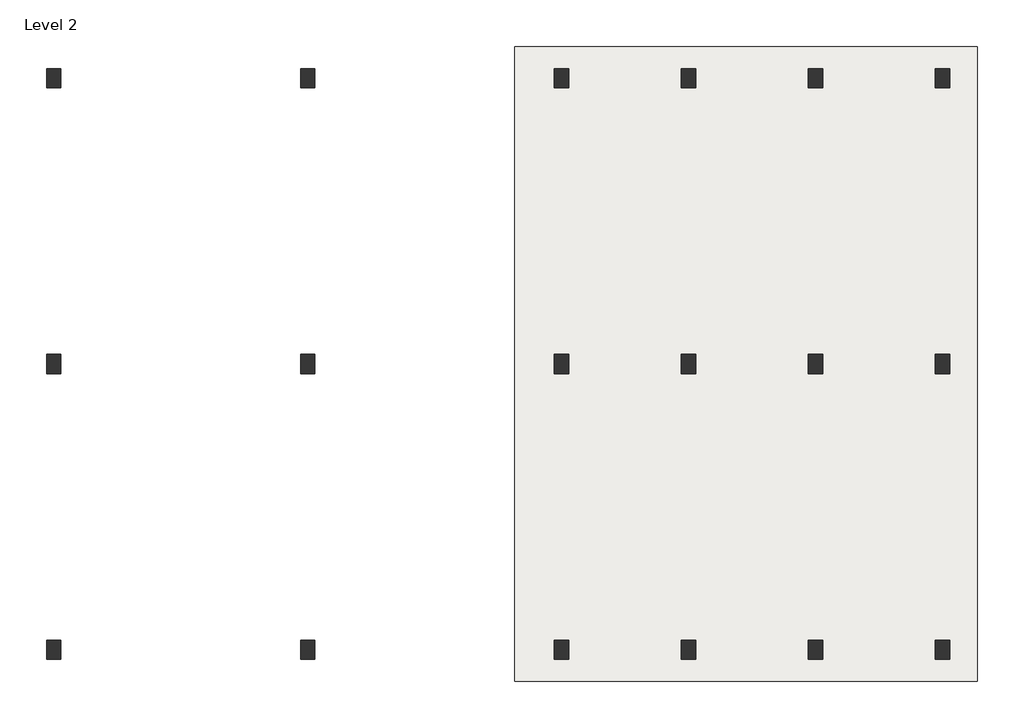
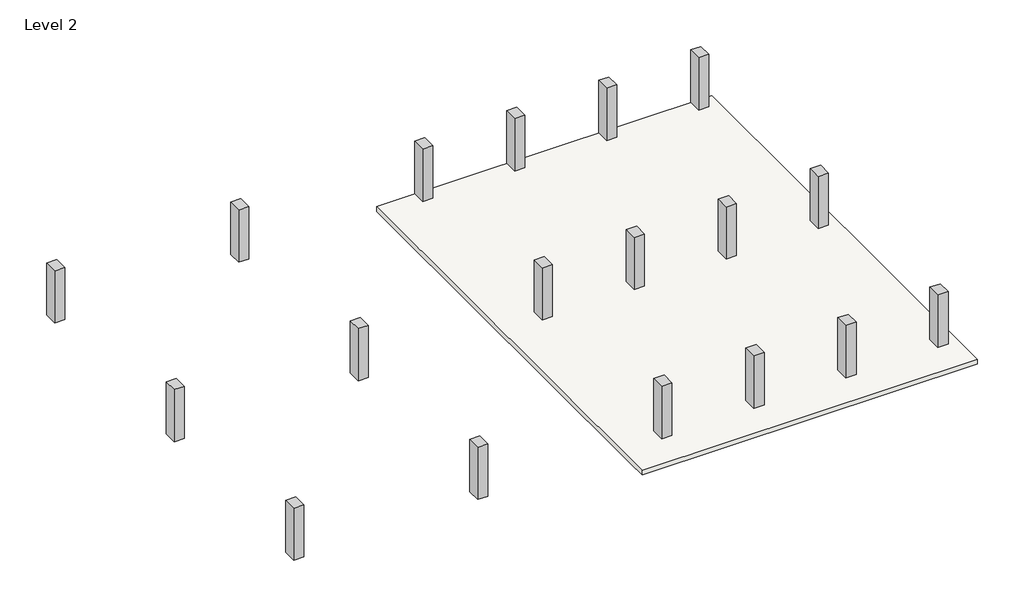
# One storey: 18 columns, 1 slab.
"""IFC4 building model written with IfcOpenShell, lengths in millimetres."""

import ifcopenshell
import ifcopenshell.guid

model = None  # the IFC model being written
_history = None  # IfcOwnerHistory: only IFC2X3 demands one
_inside = {}  # id of a spatial element -> (the spatial element, [elements in it])
_under = {}  # id of a project, library or spatial element -> (it, [spatial elements below it])
_declared = {}  # id of a project -> (the project, [libraries it declares])
_typed = {}  # id of a type object -> (the type object, [elements of that type])
_made_of = {}  # id of a material, layer set ... -> (it, [elements and type objects made of it])


def new_model(schema):
    """Start an empty IFC model of exactly this schema.

    Asked for "IFC4X3", IfcOpenShell would pick the latest addendum, in which some entities
    have other attributes; the version numbers below select the first issue.
    IFC2X3 requires an IfcOwnerHistory on every rooted entity: one is made here for all.
    """
    global model, _history
    if schema == "IFC4X3":
        model = ifcopenshell.file(schema_version=(4, 3, 0, 0))
    else:
        model = ifcopenshell.file(schema=schema)
    _inside.clear()
    _under.clear()
    _declared.clear()
    _typed.clear()
    _made_of.clear()
    _history = None
    if model.schema == "IFC2X3":
        org = make("IfcOrganization", Name="unknown")
        user = make(
            "IfcPersonAndOrganization",
            ThePerson=make("IfcPerson", FamilyName="unknown"),
            TheOrganization=org,
        )
        app = make(
            "IfcApplication",
            ApplicationDeveloper=org,
            Version="unknown",
            ApplicationFullName="unknown",
            ApplicationIdentifier="unknown",
        )
        _history = make(
            "IfcOwnerHistory",
            OwningUser=user,
            OwningApplication=app,
            ChangeAction="ADDED",
            CreationDate=0,
        )
    return model


def make(cls, **values):
    """One entity of the class cls with the attributes given. An attribute that is None is left unset."""
    return model.create_entity(
        cls, **{name: value for name, value in values.items() if value is not None}
    )


def rooted(cls, **values):
    """An entity with a GlobalId (a new one), such as an element, a storey or a relation."""
    return make(cls, GlobalId=ifcopenshell.guid.new(), OwnerHistory=_history, **values)


def si_unit(unit_type, name, prefix=None):
    """IfcSIUnit, for example si_unit("LENGTHUNIT", "METRE", prefix="MILLI")."""
    return make("IfcSIUnit", UnitType=unit_type, Prefix=prefix, Name=name)


def assignment(units):
    """IfcUnitAssignment: the units of a project."""
    return None if units is None else make("IfcUnitAssignment", Units=units)


def point(xyz):
    """IfcCartesianPoint."""
    return None if xyz is None else make("IfcCartesianPoint", Coordinates=xyz)


def direction(xyz):
    """IfcDirection."""
    return None if xyz is None else make("IfcDirection", DirectionRatios=xyz)


def frame(location, z_axis=None, x_axis=None):
    """IfcAxis2Placement3D, a coordinate frame: its origin and axes. An axis left out is left unset."""
    return make(
        "IfcAxis2Placement3D",
        Location=point(location),
        Axis=direction(z_axis),
        RefDirection=direction(x_axis),
    )


def origin():
    """The frame at (0, 0, 0) with its axes left unset."""
    return frame((0.0, 0.0, 0.0))


def place(relative_to, where):
    """IfcLocalPlacement: puts the frame where relative to a parent placement (None: the world)."""
    return make(
        "IfcLocalPlacement", PlacementRelTo=relative_to, RelativePlacement=where
    )


def context(
    kind, dimensions, precision=None, world=None, true_north=None, identifier=None
):
    """IfcGeometricRepresentationContext, for example the 3D "Model" context."""
    return make(
        "IfcGeometricRepresentationContext",
        ContextIdentifier=identifier,
        ContextType=kind,
        CoordinateSpaceDimension=dimensions,
        Precision=precision,
        WorldCoordinateSystem=world,
        TrueNorth=true_north,
    )


def project(units=None, contexts=None):
    """IfcProject with its units and contexts."""
    return rooted(
        "IfcProject",
        Name="project",
        RepresentationContexts=contexts,
        UnitsInContext=assignment(units),
    )


def spatial(cls, under=None, at=None, **own):
    """A site, building, storey or space (cls), placed at a placement, below another one or the project."""
    s = rooted(cls, ObjectPlacement=at, **own)
    if under is not None:
        _under.setdefault(under.id(), (under, []))[1].append(s)
    return s


def polyline(points):
    """IfcPolyline through the points."""
    return make("IfcPolyline", Points=[point(p) for p in points])


def outline(outer, holes=None, kind="AREA"):
    """IfcArbitraryClosedProfileDef: a profile drawn as a closed curve; with holes, ...WithVoids."""
    if holes is None:
        return make("IfcArbitraryClosedProfileDef", ProfileType=kind, OuterCurve=outer)
    return make(
        "IfcArbitraryProfileDefWithVoids",
        ProfileType=kind,
        OuterCurve=outer,
        InnerCurves=holes,
    )


def extrude(swept, where, along, depth):
    """IfcExtrudedAreaSolid: the profile swept, set in the frame where, extruded along a direction by depth."""
    return make(
        "IfcExtrudedAreaSolid",
        SweptArea=swept,
        Position=where,
        ExtrudedDirection=direction(along),
        Depth=depth,
    )


def faces_of(points, faces, orient=None, outer=None):
    """IfcFace entities. A face is a list of loops; a loop is a list of indices into points, from 0.

    orient and outer hold one flag for each loop. By default every Orientation is true, the
    first loop of a face is its IfcFaceOuterBound and the others are IfcFaceBound.
    """
    made = []
    for i, loops in enumerate(faces):
        bounds = []
        for j, loop in enumerate(loops):
            is_outer = j == 0 if outer is None else outer[i][j]
            bounds.append(
                make(
                    "IfcFaceOuterBound" if is_outer else "IfcFaceBound",
                    Bound=make("IfcPolyLoop", Polygon=[points[k] for k in loop]),
                    Orientation=True if orient is None else orient[i][j],
                )
            )
        made.append(make("IfcFace", Bounds=bounds))
    return made


def faceted_brep(points, faces, orient=None, outer=None, voids=None):
    """IfcFacetedBrep: a solid bounded by flat faces; with voids (closed shells), ...WithVoids."""
    shared = [point(p) for p in points]
    hull = make("IfcClosedShell", CfsFaces=faces_of(shared, faces, orient, outer))
    if voids is None:
        return make("IfcFacetedBrep", Outer=hull)
    return make(
        "IfcFacetedBrepWithVoids",
        Outer=hull,
        Voids=[
            make(cls, CfsFaces=faces_of(shared, fs, o, b)) for cls, fs, o, b in voids
        ],
    )


def shape(context_of_items, identifier, shape_type, items):
    """IfcShapeRepresentation: the items that make up one representation, for example the "Body"."""
    return make(
        "IfcShapeRepresentation",
        ContextOfItems=context_of_items,
        RepresentationIdentifier=identifier,
        RepresentationType=shape_type,
        Items=items,
    )


def source(mapping_origin, context_of_items, identifier, shape_type, items):
    """IfcRepresentationMap: a shape defined once, which mapped items show again and again."""
    return make(
        "IfcRepresentationMap",
        MappingOrigin=mapping_origin,
        MappedRepresentation=shape(context_of_items, identifier, shape_type, items),
    )


def transform(
    local_origin,
    x_axis=None,
    y_axis=None,
    z_axis=None,
    scale=None,
    scale2=None,
    scale3=None,
    uniform=True,
):
    """IfcCartesianTransformationOperator3D, or its non-uniform kind. x_axis, y_axis, z_axis: its Axis1, 2, 3."""
    if uniform:
        return make(
            "IfcCartesianTransformationOperator3D",
            Axis1=direction(x_axis),
            Axis2=direction(y_axis),
            LocalOrigin=point(local_origin),
            Scale=scale,
            Axis3=direction(z_axis),
        )
    return make(
        "IfcCartesianTransformationOperator3DnonUniform",
        Axis1=direction(x_axis),
        Axis2=direction(y_axis),
        LocalOrigin=point(local_origin),
        Scale=scale,
        Axis3=direction(z_axis),
        Scale2=scale2,
        Scale3=scale3,
    )


def mapped(mapping_source, mapping_target):
    """IfcMappedItem: shows the shape of a source again, moved by a transform."""
    return make(
        "IfcMappedItem", MappingSource=mapping_source, MappingTarget=mapping_target
    )


def made_of(thing, what):
    """Note that an element or type object is made of a material, layer set ...; save() writes the relation."""
    if what is not None:
        _made_of.setdefault(what.id(), (what, []))[1].append(thing)
    return thing


def element(
    cls,
    number,
    at=None,
    inside=None,
    cuts=None,
    type_object=None,
    material=None,
    context=None,
    identifier="Body",
    shape_type=None,
    held_by="IfcProductDefinitionShape",
    body=None,
    shapes=None,
    **own,
):
    """One element of the class cls, such as IfcWall. Its Tag is "e" and its number.

    at: its placement. inside: the storey or other place that contains it. cuts: it is an
    opening in that element (IfcRelVoidsElement). A single representation is given by context,
    identifier, shape_type and body (its items); several are given by shapes. held_by: the class
    of the entity that holds the representations. save() writes the other relations.
    """
    e = rooted(cls, Tag="e%d" % number, ObjectPlacement=at, **own)
    if body is not None:
        shapes = [shape(context, identifier, shape_type, body)]
    if shapes is not None:
        e.Representation = make(held_by, Representations=shapes)
    if inside is not None:
        _inside.setdefault(inside.id(), (inside, []))[1].append(e)
    if cuts is not None:
        rooted(
            "IfcRelVoidsElement", RelatingBuildingElement=cuts, RelatedOpeningElement=e
        )
    if type_object is not None:
        _typed.setdefault(type_object.id(), (type_object, []))[1].append(e)
    return made_of(e, material)


def aggregate(whole, parts):
    """IfcRelAggregates: a whole, such as a stair, and the parts it consists of."""
    return rooted("IfcRelAggregates", RelatingObject=whole, RelatedObjects=parts)


def save(model, path):
    """Write the relations noted so far, then the file.

    IfcRelAggregates (storeys below a building ...), IfcRelContainedInSpatialStructure (elements
    in a storey), IfcRelDefinesByType, IfcRelAssociatesMaterial and IfcRelDeclares: one each for
    every whole, place, type object, material and project.
    """
    for whole, parts in _under.values():
        aggregate(whole, parts)
    for where, things in _inside.values():
        rooted(
            "IfcRelContainedInSpatialStructure",
            RelatedElements=things,
            RelatingStructure=where,
        )
    for kind, things in _typed.values():
        rooted("IfcRelDefinesByType", RelatedObjects=things, RelatingType=kind)
    for what, things in _made_of.values():
        rooted("IfcRelAssociatesMaterial", RelatedObjects=things, RelatingMaterial=what)
    for by, libraries in _declared.values():
        rooted("IfcRelDeclares", RelatingContext=by, RelatedDefinitions=libraries)
    model.write(path)


def concrete_rectangular_column_450_x_600mm_14788169(model_context):
    return source(origin(), model_context, "Body", "SweptSolid", [
        extrude(outline(polyline([(225.0, 300.0), (225.0, -300.0), (-225.0, -300.0), (-225.0, 300.0), (225.0, 300.0)])), frame((0.0, 0.0, 3600.0), z_axis=(0.0, 0.0, 1.0), x_axis=(1.0, 0.0, 0.0)), (0.0, 0.0, 1.0), 2400.0),
    ])


model = new_model("IFC4")

# Units and contexts
model_context = context("Model", 3, world=origin())
ifc_project = project(units=[si_unit("LENGTHUNIT", "METRE", prefix="MILLI")], contexts=[model_context])

# Site, building, storey
site = spatial("IfcSite", under=ifc_project)
building = spatial("IfcBuilding", under=site)
storey = spatial("IfcBuildingStorey", under=building, Name="Level 2", Elevation=3000.0)

# Columns
placement = place(None, origin())
element("IfcColumn", 1, ObjectType="Concrete-Rectangular-Column : 450 x 600mm", at=placement, inside=storey, context=model_context, shape_type="SweptSolid", body=[
    extrude(outline(polyline([(1008.7948332, 9883.1317199), (1008.7948332, 9283.1317199), (558.7948332, 9283.1317199), (558.7948332, 9883.1317199), (1008.7948332, 9883.1317199)])), frame((0.0, 0.0, 3600.0), z_axis=(0.0, 0.0, 1.0), x_axis=(1.0, 0.0, 0.0)), (0.0, 0.0, 1.0), 2400.0),
])
element("IfcColumn", 2, ObjectType="Concrete-Rectangular-Column : 450 x 600mm", at=placement, inside=storey, context=model_context, shape_type="SweptSolid", body=[
    extrude(outline(polyline([(5008.7948332, 9883.1317199), (5008.7948332, 9283.1317199), (4558.7948332, 9283.1317199), (4558.7948332, 9883.1317199), (5008.7948332, 9883.1317199)])), frame((0.0, 0.0, 3600.0), z_axis=(0.0, 0.0, 1.0), x_axis=(1.0, 0.0, 0.0)), (0.0, 0.0, 1.0), 2400.0),
])
element("IfcColumn", 3, ObjectType="Concrete-Rectangular-Column : 450 x 600mm", at=placement, inside=storey, context=model_context, shape_type="SweptSolid", body=[
    extrude(outline(polyline([(9008.7948332, 9883.1317199), (9008.7948332, 9283.1317199), (8558.7948332, 9283.1317199), (8558.7948332, 9883.1317199), (9008.7948332, 9883.1317199)])), frame((0.0, 0.0, 3600.0), z_axis=(0.0, 0.0, 1.0), x_axis=(1.0, 0.0, 0.0)), (0.0, 0.0, 1.0), 2400.0),
])
element("IfcColumn", 4, ObjectType="Concrete-Rectangular-Column : 450 x 600mm", at=placement, inside=storey, context=model_context, shape_type="SweptSolid", body=[
    extrude(outline(polyline([(13008.7948332, 9883.1317199), (13008.7948332, 9283.1317199), (12558.7948332, 9283.1317199), (12558.7948332, 9883.1317199), (13008.7948332, 9883.1317199)])), frame((0.0, 0.0, 3600.0), z_axis=(0.0, 0.0, 1.0), x_axis=(1.0, 0.0, 0.0)), (0.0, 0.0, 1.0), 2400.0),
])
element("IfcColumn", 5, ObjectType="Concrete-Rectangular-Column : 450 x 600mm", at=placement, inside=storey, context=model_context, shape_type="SweptSolid", body=[
    extrude(outline(polyline([(13008.7948332, 883.1317199), (13008.7948332, 283.1317199), (12558.7948332, 283.1317199), (12558.7948332, 883.1317199), (13008.7948332, 883.1317199)])), frame((0.0, 0.0, 3600.0), z_axis=(0.0, 0.0, 1.0), x_axis=(1.0, 0.0, 0.0)), (0.0, 0.0, 1.0), 2400.0),
])
element("IfcColumn", 6, ObjectType="Concrete-Rectangular-Column : 450 x 600mm", at=placement, inside=storey, context=model_context, shape_type="SweptSolid", body=[
    extrude(outline(polyline([(9008.7948332, 883.1317199), (9008.7948332, 283.1317199), (8558.7948332, 283.1317199), (8558.7948332, 883.1317199), (9008.7948332, 883.1317199)])), frame((0.0, 0.0, 3600.0), z_axis=(0.0, 0.0, 1.0), x_axis=(1.0, 0.0, 0.0)), (0.0, 0.0, 1.0), 2400.0),
])
element("IfcColumn", 7, ObjectType="Concrete-Rectangular-Column : 450 x 600mm", at=placement, inside=storey, context=model_context, shape_type="SweptSolid", body=[
    extrude(outline(polyline([(5008.7948332, 883.1317199), (5008.7948332, 283.1317199), (4558.7948332, 283.1317199), (4558.7948332, 883.1317199), (5008.7948332, 883.1317199)])), frame((0.0, 0.0, 3600.0), z_axis=(0.0, 0.0, 1.0), x_axis=(1.0, 0.0, 0.0)), (0.0, 0.0, 1.0), 2400.0),
])
element("IfcColumn", 8, ObjectType="Concrete-Rectangular-Column : 450 x 600mm", at=placement, inside=storey, context=model_context, shape_type="SweptSolid", body=[
    extrude(outline(polyline([(1008.7948332, 883.1317199), (1008.7948332, 283.1317199), (558.7948332, 283.1317199), (558.7948332, 883.1317199), (1008.7948332, 883.1317199)])), frame((0.0, 0.0, 3600.0), z_axis=(0.0, 0.0, 1.0), x_axis=(1.0, 0.0, 0.0)), (0.0, 0.0, 1.0), 2400.0),
])
element("IfcColumn", 9, ObjectType="Concrete-Rectangular-Column : 450 x 600mm", at=placement, inside=storey, context=model_context, shape_type="SweptSolid", body=[
    extrude(outline(polyline([(1008.7948332, -8116.8682801), (1008.7948332, -8716.8682801), (558.7948332, -8716.8682801), (558.7948332, -8116.8682801), (1008.7948332, -8116.8682801)])), frame((0.0, 0.0, 3600.0), z_axis=(0.0, 0.0, 1.0), x_axis=(1.0, 0.0, 0.0)), (0.0, 0.0, 1.0), 2400.0),
])
element("IfcColumn", 10, ObjectType="Concrete-Rectangular-Column : 450 x 600mm", at=placement, inside=storey, context=model_context, shape_type="SweptSolid", body=[
    extrude(outline(polyline([(5008.7948332, -8116.8682801), (5008.7948332, -8716.8682801), (4558.7948332, -8716.8682801), (4558.7948332, -8116.8682801), (5008.7948332, -8116.8682801)])), frame((0.0, 0.0, 3600.0), z_axis=(0.0, 0.0, 1.0), x_axis=(1.0, 0.0, 0.0)), (0.0, 0.0, 1.0), 2400.0),
])
element("IfcColumn", 11, ObjectType="Concrete-Rectangular-Column : 450 x 600mm", at=placement, inside=storey, context=model_context, shape_type="SweptSolid", body=[
    extrude(outline(polyline([(9008.7948332, -8116.8682801), (9008.7948332, -8716.8682801), (8558.7948332, -8716.8682801), (8558.7948332, -8116.8682801), (9008.7948332, -8116.8682801)])), frame((0.0, 0.0, 3600.0), z_axis=(0.0, 0.0, 1.0), x_axis=(1.0, 0.0, 0.0)), (0.0, 0.0, 1.0), 2400.0),
])
element("IfcColumn", 12, ObjectType="Concrete-Rectangular-Column : 450 x 600mm", at=placement, inside=storey, context=model_context, shape_type="SweptSolid", body=[
    extrude(outline(polyline([(13008.7948332, -8116.8682801), (13008.7948332, -8716.8682801), (12558.7948332, -8716.8682801), (12558.7948332, -8116.8682801), (13008.7948332, -8116.8682801)])), frame((0.0, 0.0, 3600.0), z_axis=(0.0, 0.0, 1.0), x_axis=(1.0, 0.0, 0.0)), (0.0, 0.0, 1.0), 2400.0),
])
concrete_rectangular_column_450_x_600mm_shape = concrete_rectangular_column_450_x_600mm_14788169(model_context)
element("IfcColumn", 13, ObjectType="Concrete-Rectangular-Column : 450 x 600mm", at=placement, inside=storey, context=model_context, shape_type="MappedRepresentation", body=[
    mapped(concrete_rectangular_column_450_x_600mm_shape, transform((-7216.2051668, -8416.8682801, 0.0), x_axis=(1.0, 0.0, 0.0), y_axis=(0.0, 1.0, 0.0), z_axis=(0.0, 0.0, 1.0))),
])
element("IfcColumn", 14, ObjectType="Concrete-Rectangular-Column : 450 x 600mm", at=placement, inside=storey, context=model_context, shape_type="MappedRepresentation", body=[
    mapped(concrete_rectangular_column_450_x_600mm_shape, transform((-15216.2051668, -8416.8682801, 0.0), x_axis=(1.0, 0.0, 0.0), y_axis=(0.0, 1.0, 0.0), z_axis=(0.0, 0.0, 1.0))),
])
element("IfcColumn", 15, ObjectType="Concrete-Rectangular-Column : 450 x 600mm", at=placement, inside=storey, context=model_context, shape_type="MappedRepresentation", body=[
    mapped(concrete_rectangular_column_450_x_600mm_shape, transform((-15216.2051668, 583.1317199, 0.0), x_axis=(1.0, 0.0, 0.0), y_axis=(0.0, 1.0, 0.0), z_axis=(0.0, 0.0, 1.0))),
])
element("IfcColumn", 16, ObjectType="Concrete-Rectangular-Column : 450 x 600mm", at=placement, inside=storey, context=model_context, shape_type="MappedRepresentation", body=[
    mapped(concrete_rectangular_column_450_x_600mm_shape, transform((-7216.2051668, 583.1317199, 0.0), x_axis=(1.0, 0.0, 0.0), y_axis=(0.0, 1.0, 0.0), z_axis=(0.0, 0.0, 1.0))),
])
element("IfcColumn", 17, ObjectType="Concrete-Rectangular-Column : 450 x 600mm", at=placement, inside=storey, context=model_context, shape_type="MappedRepresentation", body=[
    mapped(concrete_rectangular_column_450_x_600mm_shape, transform((-7216.2051668, 9583.1317199, 0.0), x_axis=(1.0, 0.0, 0.0), y_axis=(0.0, 1.0, 0.0), z_axis=(0.0, 0.0, 1.0))),
])
element("IfcColumn", 18, ObjectType="Concrete-Rectangular-Column : 450 x 600mm", at=placement, inside=storey, context=model_context, shape_type="MappedRepresentation", body=[
    mapped(concrete_rectangular_column_450_x_600mm_shape, transform((-15216.2051668, 9583.1317199, 0.0), x_axis=(1.0, 0.0, 0.0), y_axis=(0.0, 1.0, 0.0), z_axis=(0.0, 0.0, 1.0))),
])

# Slab
element("IfcSlab", 19, ObjectType="160mm Concrete with Corus-ComFlor 70", at=placement, inside=storey, context=model_context, shape_type="Brep", body=[
    faceted_brep([(-687.3078946, 10583.1317199, 2785.0), (13883.7948332, 10583.1317199, 2785.0), (13883.7948332, -9416.8682801, 2785.0), (-687.3078946, -9416.8682801, 2785.0), (-687.3078946, -8566.8682801, 2785.0), (-687.3078946, -8266.8682801, 2785.0), (-687.3078946, 9433.1317199, 2785.0), (-687.3078946, 9733.1317199, 2785.0), (-687.3078946, 10583.1317199, 3000.0), (-687.3078946, -9416.8682801, 3000.0), (13883.7948332, -9416.8682801, 3000.0), (13883.7948332, 10583.1317199, 3000.0)], [[[0, 1, 2, 3, 4, 5, 6, 7]], [[8, 9, 10, 11]], [[1, 0, 8, 11]], [[2, 1, 11, 10]], [[3, 2, 10, 9]], [[0, 7, 6, 5, 4, 3, 9, 8]]]),
])

save(model, "model.ifc")

# Revit data of these elements
# Type "Concrete-Rectangular-Column : 450 x 600mm"
#   b = 450 mm
#   h = 600 mm
#   Structural Material [instance default] = Concrete, Cast-in-Place gray
# Type "160mm Concrete with Corus-ComFlor 70"
#   Function = 0
#   Layers, outside or top first: 215 mm "Concrete, Cast-in-Place - C15" (function 1); 0 mm "Metal Deck" (function 200)
# Elements 1, 2, 3, 4, 5, 6, 7, 8, 9, 10, 11, 12, 13, 14, 15, 16, 17, 18 (IfcColumn, "Concrete-Rectangular-Column : 450 x 600mm")
#   Structural Material = Concrete, Cast-in-Place gray
#   Phase Created = New Construction
#   Materials on its faces: "Concrete, Cast-in-Place gray"
# Element 19 (IfcSlab, "160mm Concrete with Corus-ComFlor 70")
#   built-in parameter 1001955 = 3.14159 (stored number, unit not read)
#   Height Offset From Level = 0 mm
#   built-in parameter 1001954 = 1
#   Phase Created = New Construction
#   Materials on its faces: "Metal Deck", "Concrete, Cast-in-Place - C15"
# Materials
#   "Concrete, Cast-in-Place gray": class "Concrete", colour RGB 192 192 192, transparency 0, Description = "Cast-in-place concrete", Cost = 0
#   "Concrete, Cast-in-Place - C15": class "Concrete", colour RGB 192 192 192, transparency 0, Description = "Concrete 15 MPa", Cost = 0
#   "Metal Deck": class "Metal", colour RGB 247 247 247, transparency 0, Description = "Steel, mill finish", Cost = 0
